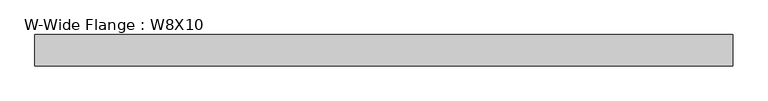
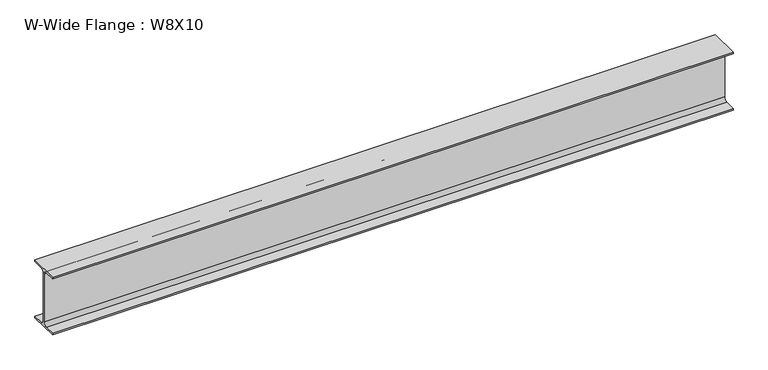
"""IFC4 building model written with IfcOpenShell, lengths in millimetres: beam geometry, W-Wide Flange : W8X10."""

import ifcopenshell
import ifcopenshell.guid

model = None  # the IFC model being written
_history = None  # IfcOwnerHistory: only IFC2X3 demands one
_inside = {}  # id of a spatial element -> (the spatial element, [elements in it])
_under = {}  # id of a project, library or spatial element -> (it, [spatial elements below it])
_declared = {}  # id of a project -> (the project, [libraries it declares])
_typed = {}  # id of a type object -> (the type object, [elements of that type])
_made_of = {}  # id of a material, layer set ... -> (it, [elements and type objects made of it])


def new_model(schema):
    """Start an empty IFC model of exactly this schema.

    Asked for "IFC4X3", IfcOpenShell would pick the latest addendum, in which some entities
    have other attributes; the version numbers below select the first issue.
    IFC2X3 requires an IfcOwnerHistory on every rooted entity: one is made here for all.
    """
    global model, _history
    if schema == "IFC4X3":
        model = ifcopenshell.file(schema_version=(4, 3, 0, 0))
    else:
        model = ifcopenshell.file(schema=schema)
    _inside.clear()
    _under.clear()
    _declared.clear()
    _typed.clear()
    _made_of.clear()
    _history = None
    if model.schema == "IFC2X3":
        org = make("IfcOrganization", Name="unknown")
        user = make(
            "IfcPersonAndOrganization",
            ThePerson=make("IfcPerson", FamilyName="unknown"),
            TheOrganization=org,
        )
        app = make(
            "IfcApplication",
            ApplicationDeveloper=org,
            Version="unknown",
            ApplicationFullName="unknown",
            ApplicationIdentifier="unknown",
        )
        _history = make(
            "IfcOwnerHistory",
            OwningUser=user,
            OwningApplication=app,
            ChangeAction="ADDED",
            CreationDate=0,
        )
    return model


def make(cls, **values):
    """One entity of the class cls with the attributes given. An attribute that is None is left unset."""
    return model.create_entity(
        cls, **{name: value for name, value in values.items() if value is not None}
    )


def rooted(cls, **values):
    """An entity with a GlobalId (a new one), such as an element, a storey or a relation."""
    return make(cls, GlobalId=ifcopenshell.guid.new(), OwnerHistory=_history, **values)


def si_unit(unit_type, name, prefix=None):
    """IfcSIUnit, for example si_unit("LENGTHUNIT", "METRE", prefix="MILLI")."""
    return make("IfcSIUnit", UnitType=unit_type, Prefix=prefix, Name=name)


def assignment(units):
    """IfcUnitAssignment: the units of a project."""
    return None if units is None else make("IfcUnitAssignment", Units=units)


def point(xyz):
    """IfcCartesianPoint."""
    return None if xyz is None else make("IfcCartesianPoint", Coordinates=xyz)


def direction(xyz):
    """IfcDirection."""
    return None if xyz is None else make("IfcDirection", DirectionRatios=xyz)


def frame(location, z_axis=None, x_axis=None):
    """IfcAxis2Placement3D, a coordinate frame: its origin and axes. An axis left out is left unset."""
    return make(
        "IfcAxis2Placement3D",
        Location=point(location),
        Axis=direction(z_axis),
        RefDirection=direction(x_axis),
    )


def frame_2d(location, x_axis=None):
    """IfcAxis2Placement2D, a coordinate frame in the plane: its origin and x axis."""
    return make(
        "IfcAxis2Placement2D", Location=point(location), RefDirection=direction(x_axis)
    )


def origin():
    """The frame at (0, 0, 0) with its axes left unset."""
    return frame((0.0, 0.0, 0.0))


def place(relative_to, where):
    """IfcLocalPlacement: puts the frame where relative to a parent placement (None: the world)."""
    return make(
        "IfcLocalPlacement", PlacementRelTo=relative_to, RelativePlacement=where
    )


def context(
    kind, dimensions, precision=None, world=None, true_north=None, identifier=None
):
    """IfcGeometricRepresentationContext, for example the 3D "Model" context."""
    return make(
        "IfcGeometricRepresentationContext",
        ContextIdentifier=identifier,
        ContextType=kind,
        CoordinateSpaceDimension=dimensions,
        Precision=precision,
        WorldCoordinateSystem=world,
        TrueNorth=true_north,
    )


def project(units=None, contexts=None):
    """IfcProject with its units and contexts."""
    return rooted(
        "IfcProject",
        Name="project",
        RepresentationContexts=contexts,
        UnitsInContext=assignment(units),
    )


def spatial(cls, under=None, at=None, **own):
    """A site, building, storey or space (cls), placed at a placement, below another one or the project."""
    s = rooted(cls, ObjectPlacement=at, **own)
    if under is not None:
        _under.setdefault(under.id(), (under, []))[1].append(s)
    return s


def polyline(points):
    """IfcPolyline through the points."""
    return make("IfcPolyline", Points=[point(p) for p in points])


def circle_curve(where, radius):
    """IfcCircle in the frame where."""
    return make("IfcCircle", Position=where, Radius=radius)


def trimmed(basis, trim1, trim2, sense, master):
    """IfcTrimmedCurve: the piece of a basis curve between two trims."""
    return make(
        "IfcTrimmedCurve",
        BasisCurve=basis,
        Trim1=trim1,
        Trim2=trim2,
        SenseAgreement=sense,
        MasterRepresentation=master,
    )


def segment(curve, same_sense, transition):
    """IfcCompositeCurveSegment."""
    return make(
        "IfcCompositeCurveSegment",
        Transition=transition,
        SameSense=same_sense,
        ParentCurve=curve,
    )


def composite_curve(segments, self_intersect=None):
    """IfcCompositeCurve: segments joined end to end."""
    return make("IfcCompositeCurve", Segments=segments, SelfIntersect=self_intersect)


def outline(outer, holes=None, kind="AREA"):
    """IfcArbitraryClosedProfileDef: a profile drawn as a closed curve; with holes, ...WithVoids."""
    if holes is None:
        return make("IfcArbitraryClosedProfileDef", ProfileType=kind, OuterCurve=outer)
    return make(
        "IfcArbitraryProfileDefWithVoids",
        ProfileType=kind,
        OuterCurve=outer,
        InnerCurves=holes,
    )


def extrude(swept, where, along, depth):
    """IfcExtrudedAreaSolid: the profile swept, set in the frame where, extruded along a direction by depth."""
    return make(
        "IfcExtrudedAreaSolid",
        SweptArea=swept,
        Position=where,
        ExtrudedDirection=direction(along),
        Depth=depth,
    )


def shape(context_of_items, identifier, shape_type, items):
    """IfcShapeRepresentation: the items that make up one representation, for example the "Body"."""
    return make(
        "IfcShapeRepresentation",
        ContextOfItems=context_of_items,
        RepresentationIdentifier=identifier,
        RepresentationType=shape_type,
        Items=items,
    )


def source(mapping_origin, context_of_items, identifier, shape_type, items):
    """IfcRepresentationMap: a shape defined once, which mapped items show again and again."""
    return make(
        "IfcRepresentationMap",
        MappingOrigin=mapping_origin,
        MappedRepresentation=shape(context_of_items, identifier, shape_type, items),
    )


def transform(
    local_origin,
    x_axis=None,
    y_axis=None,
    z_axis=None,
    scale=None,
    scale2=None,
    scale3=None,
    uniform=True,
):
    """IfcCartesianTransformationOperator3D, or its non-uniform kind. x_axis, y_axis, z_axis: its Axis1, 2, 3."""
    if uniform:
        return make(
            "IfcCartesianTransformationOperator3D",
            Axis1=direction(x_axis),
            Axis2=direction(y_axis),
            LocalOrigin=point(local_origin),
            Scale=scale,
            Axis3=direction(z_axis),
        )
    return make(
        "IfcCartesianTransformationOperator3DnonUniform",
        Axis1=direction(x_axis),
        Axis2=direction(y_axis),
        LocalOrigin=point(local_origin),
        Scale=scale,
        Axis3=direction(z_axis),
        Scale2=scale2,
        Scale3=scale3,
    )


def mapped(mapping_source, mapping_target):
    """IfcMappedItem: shows the shape of a source again, moved by a transform."""
    return make(
        "IfcMappedItem", MappingSource=mapping_source, MappingTarget=mapping_target
    )


def made_of(thing, what):
    """Note that an element or type object is made of a material, layer set ...; save() writes the relation."""
    if what is not None:
        _made_of.setdefault(what.id(), (what, []))[1].append(thing)
    return thing


def element(
    cls,
    number,
    at=None,
    inside=None,
    cuts=None,
    type_object=None,
    material=None,
    context=None,
    identifier="Body",
    shape_type=None,
    held_by="IfcProductDefinitionShape",
    body=None,
    shapes=None,
    **own,
):
    """One element of the class cls, such as IfcWall. Its Tag is "e" and its number.

    at: its placement. inside: the storey or other place that contains it. cuts: it is an
    opening in that element (IfcRelVoidsElement). A single representation is given by context,
    identifier, shape_type and body (its items); several are given by shapes. held_by: the class
    of the entity that holds the representations. save() writes the other relations.
    """
    e = rooted(cls, Tag="e%d" % number, ObjectPlacement=at, **own)
    if body is not None:
        shapes = [shape(context, identifier, shape_type, body)]
    if shapes is not None:
        e.Representation = make(held_by, Representations=shapes)
    if inside is not None:
        _inside.setdefault(inside.id(), (inside, []))[1].append(e)
    if cuts is not None:
        rooted(
            "IfcRelVoidsElement", RelatingBuildingElement=cuts, RelatedOpeningElement=e
        )
    if type_object is not None:
        _typed.setdefault(type_object.id(), (type_object, []))[1].append(e)
    return made_of(e, material)


def aggregate(whole, parts):
    """IfcRelAggregates: a whole, such as a stair, and the parts it consists of."""
    return rooted("IfcRelAggregates", RelatingObject=whole, RelatedObjects=parts)


def save(model, path):
    """Write the relations noted so far, then the file.

    IfcRelAggregates (storeys below a building ...), IfcRelContainedInSpatialStructure (elements
    in a storey), IfcRelDefinesByType, IfcRelAssociatesMaterial and IfcRelDeclares: one each for
    every whole, place, type object, material and project.
    """
    for whole, parts in _under.values():
        aggregate(whole, parts)
    for where, things in _inside.values():
        rooted(
            "IfcRelContainedInSpatialStructure",
            RelatedElements=things,
            RelatingStructure=where,
        )
    for kind, things in _typed.values():
        rooted("IfcRelDefinesByType", RelatedObjects=things, RelatingType=kind)
    for what, things in _made_of.values():
        rooted("IfcRelAssociatesMaterial", RelatedObjects=things, RelatingMaterial=what)
    for by, libraries in _declared.values():
        rooted("IfcRelDeclares", RelatingContext=by, RelatedDefinitions=libraries)
    model.write(path)


def w_wide_flange_w8x10_c8dde3b0(model_context):
    return source(origin(), model_context, "Body", "SweptSolid", [
        extrude(outline(composite_curve([segment(polyline([(50.038, -94.996), (50.038, -100.203), (-50.038, -100.203), (-50.038, -94.996), (-14.4145, -94.996)]), True, "CONTINUOUS"), segment(trimmed(circle_curve(frame_2d((-14.4145, -82.7405)), 12.2555), [point((-14.4145, -94.996))], [point((-2.159, -82.7405))], True, "CARTESIAN"), True, "CONTINUOUS"), segment(polyline([(-2.159, -82.7405), (-2.159, 82.7405)]), True, "CONTINUOUS"), segment(trimmed(circle_curve(frame_2d((-14.4145, 82.7405)), 12.2555), [point((-2.159, 82.7405))], [point((-14.4145, 94.996))], True, "CARTESIAN"), True, "CONTINUOUS"), segment(polyline([(-14.4145, 94.996), (-50.038, 94.996), (-50.038, 100.203), (50.038, 100.203), (50.038, 94.996), (14.4145, 94.996)]), True, "CONTINUOUS"), segment(trimmed(circle_curve(frame_2d((14.4145, 82.7405)), 12.2555), [point((14.4145, 94.996))], [point((2.159, 82.7405))], True, "CARTESIAN"), True, "CONTINUOUS"), segment(polyline([(2.159, 82.7405), (2.159, -82.7405)]), True, "CONTINUOUS"), segment(trimmed(circle_curve(frame_2d((14.4145, -82.7405)), 12.2555), [point((2.159, -82.7405))], [point((14.4145, -94.996))], True, "CARTESIAN"), True, "CONTINUOUS"), segment(polyline([(14.4145, -94.996), (50.038, -94.996)]), True, "CONTINUOUS")], self_intersect=False)), frame((-1117.6, 0.0, 0.0), z_axis=(1.0, 0.0, 0.0), x_axis=(0.0, 1.0, 0.0)), (0.0, 0.0, 1.0), 2235.2),
    ])


if __name__ == "__main__":
    model = new_model("IFC4")
    model_context = context("Model", 3, world=origin())
    ifc_project = project(units=[si_unit("LENGTHUNIT", "METRE", prefix="MILLI")], contexts=[model_context])
    site = spatial("IfcSite", under=ifc_project)
    building = spatial("IfcBuilding", under=site)
    placement = place(None, origin())
    w_wide_flange_w8x10_shape = w_wide_flange_w8x10_c8dde3b0(model_context)
    element("IfcBeam", 1, ObjectType="W-Wide Flange : W8X10", at=placement, inside=building, context=model_context, shape_type="MappedRepresentation", body=[
        mapped(w_wide_flange_w8x10_shape, transform((0.0, 0.0, 0.0), x_axis=(1.0, 0.0, 0.0), y_axis=(0.0, 1.0, 0.0), z_axis=(0.0, 0.0, 1.0))),
    ])
    save(model, "model.ifc")

# Revit data of these elements
# Type "W-Wide Flange : W8X10"
#   Assembly Code = "B10"
#   W = 10
#   Length [instance default] = 5' - 0"
#   bf = 0' - 3.94"
#   d = 0' - 7.89"
#   k = 0' - 0 11/16"
#   k2 = 0' - 0.4825"
#   tf = 0' - 0.205"
#   tw = 0' - 0.17"
#   A = 0.0205556 SF
#   Structural Material [instance default] = Steel ASTM A992
# Element 1 (IfcBeam, "W-Wide Flange : W8X10")
#   Structural Material = PAINTED STEEL
#   Materials on its faces: "PAINTED STEEL"
# Materials
#   "Steel ASTM A992": class "Metal", colour RGB 189 187 185, transparency 0, Description = "Structural steel 50ksi", Cost = 0
#   "PAINTED STEEL": class "Generic", colour RGB 120 120 120, transparency 0, Cost = 0
